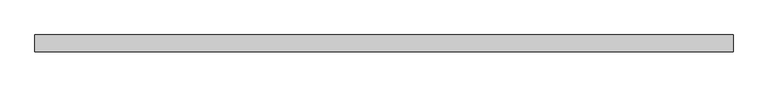
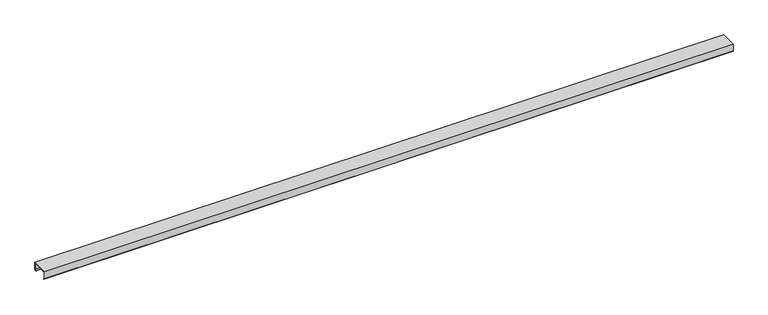
"""IFC4 building model written with IfcOpenShell, lengths in millimetres: proxy geometry, Generic Models 7:Generic Models 1:1:Generic Models 1:1 : Generic Models 7:Generic Models 1:337419:38 : Generic Models 7:Generic Models 1:1:Generic Models 1:1 : Generic Models 7:Generic Models 1:337419:306201."""

import ifcopenshell
import ifcopenshell.guid

model = None  # the IFC model being written
_history = None  # IfcOwnerHistory: only IFC2X3 demands one
_inside = {}  # id of a spatial element -> (the spatial element, [elements in it])
_under = {}  # id of a project, library or spatial element -> (it, [spatial elements below it])
_declared = {}  # id of a project -> (the project, [libraries it declares])
_typed = {}  # id of a type object -> (the type object, [elements of that type])
_made_of = {}  # id of a material, layer set ... -> (it, [elements and type objects made of it])


def new_model(schema):
    """Start an empty IFC model of exactly this schema.

    Asked for "IFC4X3", IfcOpenShell would pick the latest addendum, in which some entities
    have other attributes; the version numbers below select the first issue.
    IFC2X3 requires an IfcOwnerHistory on every rooted entity: one is made here for all.
    """
    global model, _history
    if schema == "IFC4X3":
        model = ifcopenshell.file(schema_version=(4, 3, 0, 0))
    else:
        model = ifcopenshell.file(schema=schema)
    _inside.clear()
    _under.clear()
    _declared.clear()
    _typed.clear()
    _made_of.clear()
    _history = None
    if model.schema == "IFC2X3":
        org = make("IfcOrganization", Name="unknown")
        user = make(
            "IfcPersonAndOrganization",
            ThePerson=make("IfcPerson", FamilyName="unknown"),
            TheOrganization=org,
        )
        app = make(
            "IfcApplication",
            ApplicationDeveloper=org,
            Version="unknown",
            ApplicationFullName="unknown",
            ApplicationIdentifier="unknown",
        )
        _history = make(
            "IfcOwnerHistory",
            OwningUser=user,
            OwningApplication=app,
            ChangeAction="ADDED",
            CreationDate=0,
        )
    return model


def make(cls, **values):
    """One entity of the class cls with the attributes given. An attribute that is None is left unset."""
    return model.create_entity(
        cls, **{name: value for name, value in values.items() if value is not None}
    )


def rooted(cls, **values):
    """An entity with a GlobalId (a new one), such as an element, a storey or a relation."""
    return make(cls, GlobalId=ifcopenshell.guid.new(), OwnerHistory=_history, **values)


def si_unit(unit_type, name, prefix=None):
    """IfcSIUnit, for example si_unit("LENGTHUNIT", "METRE", prefix="MILLI")."""
    return make("IfcSIUnit", UnitType=unit_type, Prefix=prefix, Name=name)


def assignment(units):
    """IfcUnitAssignment: the units of a project."""
    return None if units is None else make("IfcUnitAssignment", Units=units)


def point(xyz):
    """IfcCartesianPoint."""
    return None if xyz is None else make("IfcCartesianPoint", Coordinates=xyz)


def direction(xyz):
    """IfcDirection."""
    return None if xyz is None else make("IfcDirection", DirectionRatios=xyz)


def frame(location, z_axis=None, x_axis=None):
    """IfcAxis2Placement3D, a coordinate frame: its origin and axes. An axis left out is left unset."""
    return make(
        "IfcAxis2Placement3D",
        Location=point(location),
        Axis=direction(z_axis),
        RefDirection=direction(x_axis),
    )


def origin():
    """The frame at (0, 0, 0) with its axes left unset."""
    return frame((0.0, 0.0, 0.0))


def place(relative_to, where):
    """IfcLocalPlacement: puts the frame where relative to a parent placement (None: the world)."""
    return make(
        "IfcLocalPlacement", PlacementRelTo=relative_to, RelativePlacement=where
    )


def context(
    kind, dimensions, precision=None, world=None, true_north=None, identifier=None
):
    """IfcGeometricRepresentationContext, for example the 3D "Model" context."""
    return make(
        "IfcGeometricRepresentationContext",
        ContextIdentifier=identifier,
        ContextType=kind,
        CoordinateSpaceDimension=dimensions,
        Precision=precision,
        WorldCoordinateSystem=world,
        TrueNorth=true_north,
    )


def project(units=None, contexts=None):
    """IfcProject with its units and contexts."""
    return rooted(
        "IfcProject",
        Name="project",
        RepresentationContexts=contexts,
        UnitsInContext=assignment(units),
    )


def spatial(cls, under=None, at=None, **own):
    """A site, building, storey or space (cls), placed at a placement, below another one or the project."""
    s = rooted(cls, ObjectPlacement=at, **own)
    if under is not None:
        _under.setdefault(under.id(), (under, []))[1].append(s)
    return s


def polyline(points):
    """IfcPolyline through the points."""
    return make("IfcPolyline", Points=[point(p) for p in points])


def outline(outer, holes=None, kind="AREA"):
    """IfcArbitraryClosedProfileDef: a profile drawn as a closed curve; with holes, ...WithVoids."""
    if holes is None:
        return make("IfcArbitraryClosedProfileDef", ProfileType=kind, OuterCurve=outer)
    return make(
        "IfcArbitraryProfileDefWithVoids",
        ProfileType=kind,
        OuterCurve=outer,
        InnerCurves=holes,
    )


def extrude(swept, where, along, depth):
    """IfcExtrudedAreaSolid: the profile swept, set in the frame where, extruded along a direction by depth."""
    return make(
        "IfcExtrudedAreaSolid",
        SweptArea=swept,
        Position=where,
        ExtrudedDirection=direction(along),
        Depth=depth,
    )


def shape(context_of_items, identifier, shape_type, items):
    """IfcShapeRepresentation: the items that make up one representation, for example the "Body"."""
    return make(
        "IfcShapeRepresentation",
        ContextOfItems=context_of_items,
        RepresentationIdentifier=identifier,
        RepresentationType=shape_type,
        Items=items,
    )


def source(mapping_origin, context_of_items, identifier, shape_type, items):
    """IfcRepresentationMap: a shape defined once, which mapped items show again and again."""
    return make(
        "IfcRepresentationMap",
        MappingOrigin=mapping_origin,
        MappedRepresentation=shape(context_of_items, identifier, shape_type, items),
    )


def transform(
    local_origin,
    x_axis=None,
    y_axis=None,
    z_axis=None,
    scale=None,
    scale2=None,
    scale3=None,
    uniform=True,
):
    """IfcCartesianTransformationOperator3D, or its non-uniform kind. x_axis, y_axis, z_axis: its Axis1, 2, 3."""
    if uniform:
        return make(
            "IfcCartesianTransformationOperator3D",
            Axis1=direction(x_axis),
            Axis2=direction(y_axis),
            LocalOrigin=point(local_origin),
            Scale=scale,
            Axis3=direction(z_axis),
        )
    return make(
        "IfcCartesianTransformationOperator3DnonUniform",
        Axis1=direction(x_axis),
        Axis2=direction(y_axis),
        LocalOrigin=point(local_origin),
        Scale=scale,
        Axis3=direction(z_axis),
        Scale2=scale2,
        Scale3=scale3,
    )


def mapped(mapping_source, mapping_target):
    """IfcMappedItem: shows the shape of a source again, moved by a transform."""
    return make(
        "IfcMappedItem", MappingSource=mapping_source, MappingTarget=mapping_target
    )


def made_of(thing, what):
    """Note that an element or type object is made of a material, layer set ...; save() writes the relation."""
    if what is not None:
        _made_of.setdefault(what.id(), (what, []))[1].append(thing)
    return thing


def element(
    cls,
    number,
    at=None,
    inside=None,
    cuts=None,
    type_object=None,
    material=None,
    context=None,
    identifier="Body",
    shape_type=None,
    held_by="IfcProductDefinitionShape",
    body=None,
    shapes=None,
    **own,
):
    """One element of the class cls, such as IfcWall. Its Tag is "e" and its number.

    at: its placement. inside: the storey or other place that contains it. cuts: it is an
    opening in that element (IfcRelVoidsElement). A single representation is given by context,
    identifier, shape_type and body (its items); several are given by shapes. held_by: the class
    of the entity that holds the representations. save() writes the other relations.
    """
    e = rooted(cls, Tag="e%d" % number, ObjectPlacement=at, **own)
    if body is not None:
        shapes = [shape(context, identifier, shape_type, body)]
    if shapes is not None:
        e.Representation = make(held_by, Representations=shapes)
    if inside is not None:
        _inside.setdefault(inside.id(), (inside, []))[1].append(e)
    if cuts is not None:
        rooted(
            "IfcRelVoidsElement", RelatingBuildingElement=cuts, RelatedOpeningElement=e
        )
    if type_object is not None:
        _typed.setdefault(type_object.id(), (type_object, []))[1].append(e)
    return made_of(e, material)


def aggregate(whole, parts):
    """IfcRelAggregates: a whole, such as a stair, and the parts it consists of."""
    return rooted("IfcRelAggregates", RelatingObject=whole, RelatedObjects=parts)


def save(model, path):
    """Write the relations noted so far, then the file.

    IfcRelAggregates (storeys below a building ...), IfcRelContainedInSpatialStructure (elements
    in a storey), IfcRelDefinesByType, IfcRelAssociatesMaterial and IfcRelDeclares: one each for
    every whole, place, type object, material and project.
    """
    for whole, parts in _under.values():
        aggregate(whole, parts)
    for where, things in _inside.values():
        rooted(
            "IfcRelContainedInSpatialStructure",
            RelatedElements=things,
            RelatingStructure=where,
        )
    for kind, things in _typed.values():
        rooted("IfcRelDefinesByType", RelatedObjects=things, RelatingType=kind)
    for what, things in _made_of.values():
        rooted("IfcRelAssociatesMaterial", RelatedObjects=things, RelatingMaterial=what)
    for by, libraries in _declared.values():
        rooted("IfcRelDeclares", RelatingContext=by, RelatedDefinitions=libraries)
    model.write(path)


def generic_models_2073edd6(model_context):
    return source(origin(), model_context, "Body", "SweptSolid", [
        extrude(outline(polyline([(-578797.4913841, 4985.940625), (-578797.4913841, 4897.040625), (-578812.0845307, 4884.7955211), (-578813.870275, 4886.9236883), (-578800.2695091, 4898.336086), (-578800.2695091, 4983.1625), (-578997.9132591, 4983.1625), (-578997.9132591, 4898.336086), (-578984.3124931, 4886.9236883), (-578986.0982374, 4884.7955211), (-579000.6913841, 4897.040625), (-579000.6913841, 4985.940625), (-578797.4913841, 4985.940625)])), frame((795954.8382438, 0.0, 0.0), z_axis=(1.0, 0.0, 0.0), x_axis=(0.0, 1.0, 0.0)), (0.0, 0.0, 1.0), 8480.4630788),
    ])


if __name__ == "__main__":
    model = new_model("IFC4")
    model_context = context("Model", 3, world=origin())
    ifc_project = project(units=[si_unit("LENGTHUNIT", "METRE", prefix="MILLI")], contexts=[model_context])
    site = spatial("IfcSite", under=ifc_project)
    building = spatial("IfcBuilding", under=site)
    placement = place(None, origin())
    generic_models_shape = generic_models_2073edd6(model_context)
    element("IfcBuildingElementProxy", 1, Name="Generic Models 7:Generic Models 1:1:Generic Models 1:1 : Generic Models 7:Generic Models 1:337419:38 : Generic Models 7:Generic Models 1:1:Generic Models 1:1 : Generic Models 7:Generic Models 1:337419:306201", ObjectType="Generic Models 7:Generic Models 1:1:Generic Models 1:1 : Generic Models 7:Generic Models 1:337419:38 : Generic Models 7:Generic Models 1:1:Generic Models 1:1 : Generic Models 7:Generic Models 1:337419:306201", at=placement, inside=building, context=model_context, shape_type="MappedRepresentation", body=[
        mapped(generic_models_shape, transform((0.0, 0.0, 0.0), x_axis=(1.0, 0.0, 0.0), y_axis=(0.0, 1.0, 0.0), z_axis=(0.0, 0.0, 1.0))),
    ])
    save(model, "model.ifc")

# Revit data of these elements
# Type "Generic Models 7:Generic Models 1:1:Generic Models 1:1 : Generic Models 7:Generic Models 1:337419:38 : Generic Models 7:Generic Models 1:1:Generic Models 1:1 : Generic Models 7:Generic Models 1:337419:306201"
#   NameOverride = "Generic Models 7:Generic Models 1:1:Generic Models 1:1 : Generic Models 7:Generic Models 1:337419:306201"
#   ObjectTypeOverride = "Generic Models 1:1 : Generic Models 7:Generic Models 1:337419"
#   Reference = "Generic Models 1"
#   Tag = "306201"
# Element 1 (IfcBuildingElementProxy, "Generic Models 7:Generic Models 1:1:Generic Models 1:1 : Generic Models 7:Generic Models 1:337419:38 : Generic Models 7:Generic Models 1:1:Generic Models 1:1 : Generic Models 7:Generic Models 1:337419:306201")
#   Materials on its faces: "'ZEE' SECTION (8.0x3.5Z - SEE STRUCT. DWGS)"
# Materials
#   "'ZEE' SECTION (8.0x3.5Z - SEE STRUCT. DWGS)": class "Unassigned", colour RGB 210 209 208, transparency 0, Keynote = "M05121300.02", Cost = 0
